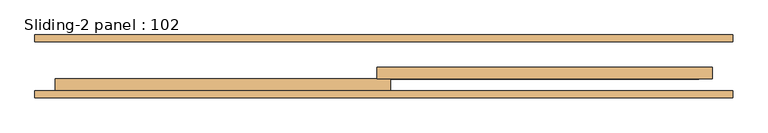
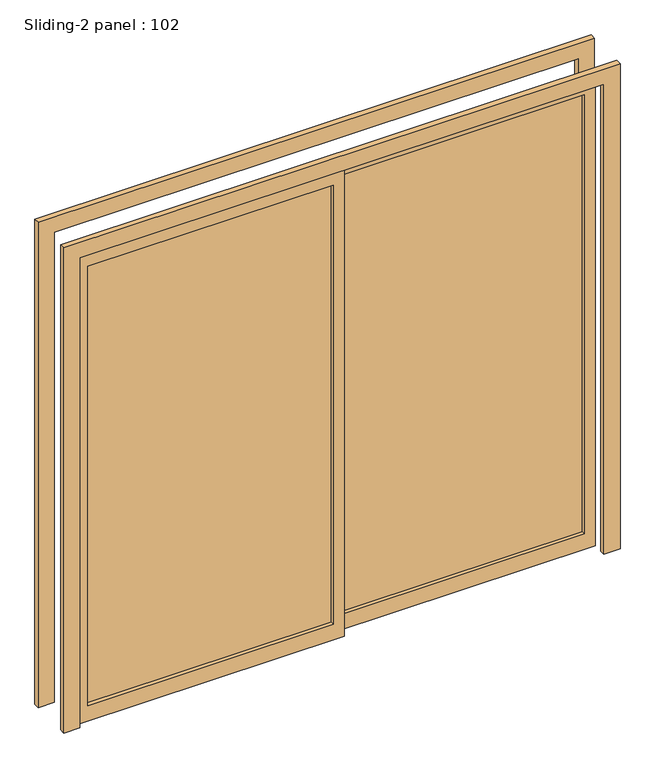
"""IFC4 building model written with IfcOpenShell, lengths in millimetres: door geometry, Sliding-2 panel : 102."""

from ifc_helpers import new_model, si_unit, frame, origin, place, context, project, spatial, polyline, outline, extrude, source, transform, mapped, element, save


def sliding_2_panel_102_1a9789c1(model_context):
    return source(origin(), model_context, "Body", "SweptSolid", [
        extrude(outline(polyline([(25.4, -155.575), (25.4, -149.225), (1181.1, -149.225), (1181.1, -155.575), (25.4, -155.575)])), frame((0.0, 0.0, 76.2), z_axis=(0.0, 0.0, 1.0), x_axis=(1.0, 0.0, 0.0)), (0.0, 0.0, 1.0), 2184.4),
        extrude(outline(polyline([(2336.8, -25.4), (0.0, -25.4), (0.0, 1231.9), (2336.8, 1231.9), (2336.8, -25.4)]), holes=[polyline([(2260.6, 25.4), (2260.6, 1181.1), (76.2, 1181.1), (76.2, 25.4), (2260.6, 25.4)])]), frame((0.0, -174.625, 0.0), z_axis=(0.0, 1.0, 0.0), x_axis=(0.0, 0.0, 1.0)), (0.0, 0.0, 1.0), 44.45),
        extrude(outline(polyline([(-1181.1, -200.025), (-1181.1, -193.675), (-25.4, -193.675), (-25.4, -200.025), (-1181.1, -200.025)])), frame((0.0, 0.0, 76.2), z_axis=(0.0, 0.0, 1.0), x_axis=(1.0, 0.0, 0.0)), (0.0, 0.0, 1.0), 2184.4),
        extrude(outline(polyline([(2336.8, 25.4), (2336.8, -1231.9), (0.0, -1231.9), (0.0, 25.4), (2336.8, 25.4)]), holes=[polyline([(2260.6, -25.4), (76.2, -25.4), (76.2, -1181.1), (2260.6, -1181.1), (2260.6, -25.4)])]), frame((0.0, -219.075, 0.0), z_axis=(0.0, 1.0, 0.0), x_axis=(0.0, 0.0, 1.0)), (0.0, 0.0, 1.0), 44.45),
        extrude(outline(polyline([(0.0, -1308.1), (0.0, -1231.9), (2336.8, -1231.9), (2336.8, 1231.9), (0.0, 1231.9), (0.0, 1308.1), (2413.0, 1308.1), (2413.0, -1308.1), (0.0, -1308.1)])), frame((0.0, -34.925, 0.0), z_axis=(0.0, 1.0, 0.0), x_axis=(0.0, 0.0, 1.0)), (0.0, 0.0, 1.0), 25.4),
        extrude(outline(polyline([(0.0, 1308.1), (2413.0, 1308.1), (2413.0, -1308.1), (0.0, -1308.1), (0.0, -1231.9), (2336.8, -1231.9), (2336.8, 1231.9), (0.0, 1231.9), (0.0, 1308.1)])), frame((0.0, -244.475, 0.0), z_axis=(0.0, 1.0, 0.0), x_axis=(0.0, 0.0, 1.0)), (0.0, 0.0, 1.0), 25.4),
    ])


if __name__ == "__main__":
    model = new_model("IFC4")
    model_context = context("Model", 3, world=origin())
    ifc_project = project(units=[si_unit("LENGTHUNIT", "METRE", prefix="MILLI")], contexts=[model_context])
    site = spatial("IfcSite", under=ifc_project)
    building = spatial("IfcBuilding", under=site)
    placement = place(None, origin())
    sliding_2_panel_102_shape = sliding_2_panel_102_1a9789c1(model_context)
    element("IfcDoor", 1, ObjectType="Sliding-2 panel : 102", at=placement, inside=building, context=model_context, shape_type="MappedRepresentation", body=[
        mapped(sliding_2_panel_102_shape, transform((0.0, 0.0, 0.0), x_axis=(1.0, 0.0, 0.0), y_axis=(0.0, 1.0, 0.0), z_axis=(0.0, 0.0, 1.0))),
    ])
    save(model, "model.ifc")

# Revit data of these elements
# Type "Sliding-2 panel : 102"
#   Type Mark = "102"
#   Construction Type Id = "MDOOR"
#   Assembly Code = "C1020"
#   Analytic Construction = "Metal"
#   Thickness = 0' - 1 3/4"
#   Heat Transfer Coefficient (U) = 3.7021 W/(m²·K)
#   Height = 7' - 8"
#   Rail Width = 0' - 3"
#   Stile Width = 0' - 2"
#   Trim Projection Ext = 0' - 1"
#   Trim Projection Int = 0' - 1"
#   Trim Width = 0' - 3"
#   Width = 8' - 1"
#   Door Material = 05 - Metal - Aluminum
#   Frame Material = 05 - Metal - Steel
#   Visual Light Transmittance = 0
#   Solar Heat Gain Coefficient = 0
#   Function = (empty or 0)
#   Wall Closure = (empty or 0)
# Element 1 (IfcDoor, "Sliding-2 panel : 102")
#   Materials on its faces: "05 - Metal - Aluminum", "05 - Metal - Steel", "Glass"
# Materials
#   "05 - Metal - Aluminum": class "Unassigned", colour RGB 247 247 247, transparency 0, Description = "Aluminum"
#   "05 - Metal - Steel": class "Unassigned", colour RGB 199 199 199, transparency 0, Description = "Steel"
#   "Glass": class "Unassigned", colour RGB 0 0 255, transparency 0.75
